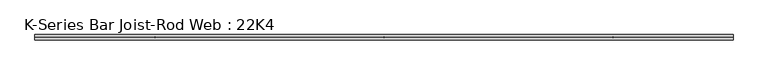
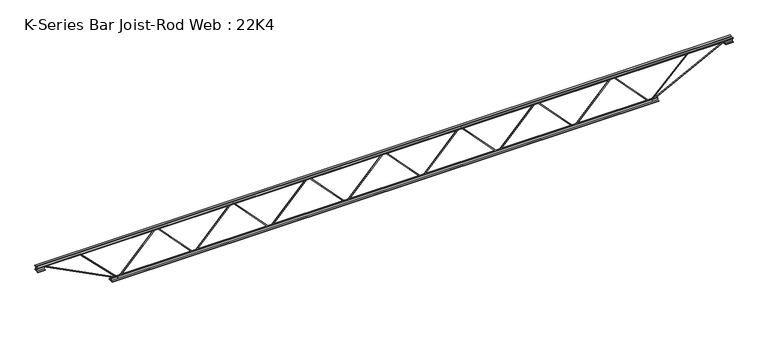
"""IFC4 building model written with IfcOpenShell, lengths in millimetres: beam geometry, K-Series Bar Joist-Rod Web : 22K4."""

from ifc_helpers import new_model, si_unit, frame, origin, place, context, project, spatial, polyline, outline, extrude, source, transform, mapped, element, save


def k_series_bar_joist_rod_web_22k4_82dcadde(model_context):
    return source(origin(), model_context, "Body", "SweptSolid", [
        extrude(outline(polyline([(-268.2875, 1561.7598214), (-277.8125, 1561.7598214), (-277.8125, 1566.9918538), (268.2875, 2081.228461), (268.2875, 2083.4643962), (-277.8125, 2597.7010033), (-277.8125, 2602.9330357), (-268.2875, 2602.9330357), (-268.2875, 2601.8150681), (277.8125, 2087.578461), (277.8125, 2077.1143962), (-268.2875, 1562.877789), (-268.2875, 1561.7598214)])), frame((0.0, -4.7625, 0.0), z_axis=(0.0, 1.0, 0.0), x_axis=(0.0, 0.0, 1.0)), (0.0, 0.0, 1.0), 9.525),
        extrude(outline(polyline([(-268.2875, 520.5866071), (-277.8125, 520.5866071), (-277.8125, 525.8186396), (268.2875, 1040.0552467), (268.2875, 1042.2911819), (-277.8125, 1556.527789), (-277.8125, 1561.7598214), (-268.2875, 1561.7598214), (-268.2875, 1560.6418538), (277.8125, 1046.4052467), (277.8125, 1035.9411819), (-268.2875, 521.7045747), (-268.2875, 520.5866071)])), frame((0.0, -4.7625, 0.0), z_axis=(0.0, 1.0, 0.0), x_axis=(0.0, 0.0, 1.0)), (0.0, 0.0, 1.0), 9.525),
        extrude(outline(polyline([(-268.2875, -520.5866071), (-277.8125, -520.5866071), (-277.8125, -515.3545747), (268.2875, -1.1179676), (268.2875, 1.1179676), (-277.8125, 515.3545747), (-277.8125, 520.5866071), (-268.2875, 520.5866071), (-268.2875, 519.4686396), (277.8125, 5.2320324), (277.8125, -5.2320324), (-268.2875, -519.4686396), (-268.2875, -520.5866071)])), frame((0.0, -4.7625, 0.0), z_axis=(0.0, 1.0, 0.0), x_axis=(0.0, 0.0, 1.0)), (0.0, 0.0, 1.0), 9.525),
        extrude(outline(polyline([(-268.2875, -1561.7598214), (-277.8125, -1561.7598214), (-277.8125, -1556.527789), (268.2875, -1042.2911819), (268.2875, -1040.0552467), (-277.8125, -525.8186396), (-277.8125, -520.5866071), (-268.2875, -520.5866071), (-268.2875, -521.7045747), (277.8125, -1035.9411819), (277.8125, -1046.4052467), (-268.2875, -1560.6418538), (-268.2875, -1561.7598214)])), frame((0.0, -4.7625, 0.0), z_axis=(0.0, 1.0, 0.0), x_axis=(0.0, 0.0, 1.0)), (0.0, 0.0, 1.0), 9.525),
        extrude(outline(polyline([(-268.2875, -2602.9330357), (-277.8125, -2602.9330357), (-277.8125, -2597.7010033), (268.2875, -2083.4643962), (268.2875, -2081.228461), (-277.8125, -1566.9918538), (-277.8125, -1561.7598214), (-268.2875, -1561.7598214), (-268.2875, -1562.877789), (277.8125, -2077.1143962), (277.8125, -2087.578461), (-268.2875, -2601.8150681), (-268.2875, -2602.9330357)])), frame((0.0, -4.7625, 0.0), z_axis=(0.0, 1.0, 0.0), x_axis=(0.0, 0.0, 1.0)), (0.0, 0.0, 1.0), 9.525),
        extrude(outline(polyline([(-268.2875, 2602.9330357), (-277.8125, 2602.9330357), (-277.8125, 2608.1650681), (268.2875, 3122.4016753), (268.2875, 3124.6376104), (-277.8125, 3638.8742176), (-277.8125, 3644.10625), (-268.2875, 3644.10625), (-268.2875, 3642.9882824), (277.8125, 3128.7516753), (277.8125, 3118.2876104), (-268.2875, 2604.0510033), (-268.2875, 2602.9330357)])), frame((0.0, -4.7625, 0.0), z_axis=(0.0, 1.0, 0.0), x_axis=(0.0, 0.0, 1.0)), (0.0, 0.0, 1.0), 9.525),
        extrude(outline(polyline([(-268.2875, -3644.10625), (-277.8125, -3644.10625), (-277.8125, -3638.8742176), (268.2875, -3124.6376104), (268.2875, -3122.4016753), (-277.8125, -2608.1650681), (-277.8125, -2602.9330357), (-268.2875, -2602.9330357), (-268.2875, -2604.0510033), (277.8125, -3118.2876104), (277.8125, -3128.7516753), (-268.2875, -3642.9882824), (-268.2875, -3644.10625)])), frame((0.0, -4.7625, 0.0), z_axis=(0.0, 1.0, 0.0), x_axis=(0.0, 0.0, 1.0)), (0.0, 0.0, 1.0), 9.525),
        extrude(outline(polyline([(4.7625, 279.4), (36.5125, 279.4), (36.5125, 273.05), (11.1125, 273.05), (11.1125, 247.65), (4.7625, 247.65), (4.7625, 279.4)])), frame((-4761.70625, 0.0, 0.0), z_axis=(1.0, 0.0, 0.0), x_axis=(0.0, 1.0, 0.0)), (0.0, 0.0, 1.0), 9523.4125),
        extrude(outline(polyline([(-4.7625, 279.4), (-4.7625, 247.65), (-11.1125, 247.65), (-11.1125, 273.05), (-36.5125, 273.05), (-36.5125, 279.4), (-4.7625, 279.4)])), frame((-4761.70625, 0.0, 0.0), z_axis=(1.0, 0.0, 0.0), x_axis=(0.0, 1.0, 0.0)), (0.0, 0.0, 1.0), 9523.4125),
        extrude(outline(polyline([(-4.7625, 215.9), (-36.5125, 215.9), (-36.5125, 222.25), (-11.1125, 222.25), (-11.1125, 247.65), (-4.7625, 247.65), (-4.7625, 215.9)])), frame((-4761.70625, 0.0, 0.0), z_axis=(1.0, 0.0, 0.0), x_axis=(0.0, 1.0, 0.0)), (0.0, 0.0, 1.0), 101.6),
        extrude(outline(polyline([(36.5125, 215.9), (4.7625, 215.9), (4.7625, 247.65), (11.1125, 247.65), (11.1125, 222.25), (36.5125, 222.25), (36.5125, 215.9)])), frame((-4761.70625, 0.0, 0.0), z_axis=(1.0, 0.0, 0.0), x_axis=(0.0, 1.0, 0.0)), (0.0, 0.0, 1.0), 101.6),
        extrude(outline(polyline([(4.7625, 215.9), (4.7625, 247.65), (11.1125, 247.65), (11.1125, 222.25), (36.5125, 222.25), (36.5125, 215.9), (4.7625, 215.9)])), frame((4660.10625, 0.0, 0.0), z_axis=(1.0, 0.0, 0.0), x_axis=(0.0, 1.0, 0.0)), (0.0, 0.0, 1.0), 101.6),
        extrude(outline(polyline([(-4.7625, 215.9), (-36.5125, 215.9), (-36.5125, 222.25), (-11.1125, 222.25), (-11.1125, 247.65), (-4.7625, 247.65), (-4.7625, 215.9)])), frame((4660.10625, 0.0, 0.0), z_axis=(1.0, 0.0, 0.0), x_axis=(0.0, 1.0, 0.0)), (0.0, 0.0, 1.0), 101.6),
        extrude(outline(polyline([(4.7625, -279.4), (4.7625, -247.65), (11.1125, -247.65), (11.1125, -273.05), (36.5125, -273.05), (36.5125, -279.4), (4.7625, -279.4)])), frame((-3745.70625, 0.0, 0.0), z_axis=(1.0, 0.0, 0.0), x_axis=(0.0, 1.0, 0.0)), (0.0, 0.0, 1.0), 7491.4125),
        extrude(outline(polyline([(-4.7625, -279.4), (-36.5125, -279.4), (-36.5125, -273.05), (-11.1125, -273.05), (-11.1125, -247.65), (-4.7625, -247.65), (-4.7625, -279.4)])), frame((-3745.70625, 0.0, 0.0), z_axis=(1.0, 0.0, 0.0), x_axis=(0.0, 1.0, 0.0)), (0.0, 0.0, 1.0), 7491.4125),
        extrude(outline(polyline([(0.0, -9.525), (0.0, 0.0), (1141.6586574, 0.0), (1141.6586574, -9.525), (0.0, -9.525)])), frame((-4662.2783824, 4.7625, 243.4116929), z_axis=(0.45609079091017707, 0.0, 0.8899332505569894), x_axis=(0.8899332505569894, 0.0, -0.45609079091017707)), (0.0, 0.0, 1.0), 9.525),
        extrude(outline(polyline([(4.7625, 4.7625), (4.7625, -4.7625), (-4.7625, -4.7625), (-4.7625, 4.7625), (4.7625, 4.7625)])), frame((-3644.10625, 0.0, -273.05), z_axis=(-0.7070297752760606, 0.0, 0.7071837787117882), x_axis=(0.0, -1.0, 0.0)), (0.0, 0.0, 1.0), 736.3008254),
        extrude(outline(polyline([(0.0, -9.525), (0.0, 0.0), (1141.6586574, 0.0), (1141.6586574, -9.525), (0.0, -9.525)])), frame((4662.2783824, -4.7625, 243.4116929), z_axis=(-0.45609079091016647, 0.0, 0.8899332505569948), x_axis=(-0.8899332505569948, 0.0, -0.45609079091016647)), (0.0, 0.0, 1.0), 9.525),
        extrude(outline(polyline([(4.7625, 4.7625), (4.7625, -4.7625), (-4.7625, -4.7625), (-4.7625, 4.7625), (4.7625, 4.7625)])), frame((3644.10625, 0.0, -273.05), z_axis=(0.7070297752760638, 0.0, 0.7071837787117848), x_axis=(0.0, -1.0, 0.0)), (0.0, 0.0, 1.0), 736.3008254),
    ])


if __name__ == "__main__":
    model = new_model("IFC4")
    model_context = context("Model", 3, world=origin())
    ifc_project = project(units=[si_unit("LENGTHUNIT", "METRE", prefix="MILLI")], contexts=[model_context])
    site = spatial("IfcSite", under=ifc_project)
    building = spatial("IfcBuilding", under=site)
    placement = place(None, origin())
    k_series_bar_joist_rod_web_22k4_shape = k_series_bar_joist_rod_web_22k4_82dcadde(model_context)
    element("IfcBeam", 1, ObjectType="K-Series Bar Joist-Rod Web : 22K4", at=placement, inside=building, context=model_context, shape_type="MappedRepresentation", body=[
        mapped(k_series_bar_joist_rod_web_22k4_shape, transform((0.0, 0.0, 0.0), x_axis=(1.0, 0.0, 0.0), y_axis=(0.0, 1.0, 0.0), z_axis=(0.0, 0.0, 1.0))),
    ])
    save(model, "model.ifc")

# Revit data of these elements
# Type "K-Series Bar Joist-Rod Web : 22K4"
#   Assembly Code = "B1010350"
#   Wt = 8
#   Web Thickness = 9.525 mm
#   Start Offset [instance default] = 0 mm
#   Start Extension [instance default] = 0 mm
#   Seat Length = 101.6 mm
#   Seat Depth = 63.5 mm
#   PanelArrayLength [instance default] = 5080 mm
#   Panel [instance default] = 1016 mm
#   End Offset [instance default] = 0 mm
#   End Extension [instance default] = 0 mm
#   End Panel = 1117.6 mm
#   Cord Leg = 31.75 mm
#   Chord Thickness = 6.35 mm
#   Length [instance default] = 7315.2 mm
#   Depth = 558.8 mm
#   PanelArrayNum [instance default] = 5
#   Structural Material = Steel ASTM A500, Grade C, Round
# Element 1 (IfcBeam, "K-Series Bar Joist-Rod Web : 22K4")
#   PanelArrayLength = 7288.212 mm
#   Panel = 1041.173 mm
#   PanelArrayNum = 7
#   Materials on its faces: "Steel ASTM A500, Grade C, Round"
# Materials
#   "Steel ASTM A500, Grade C, Round": class "Metal", colour RGB 202 101 0, transparency 0, Description = "Carbon steel", Cost = 0
